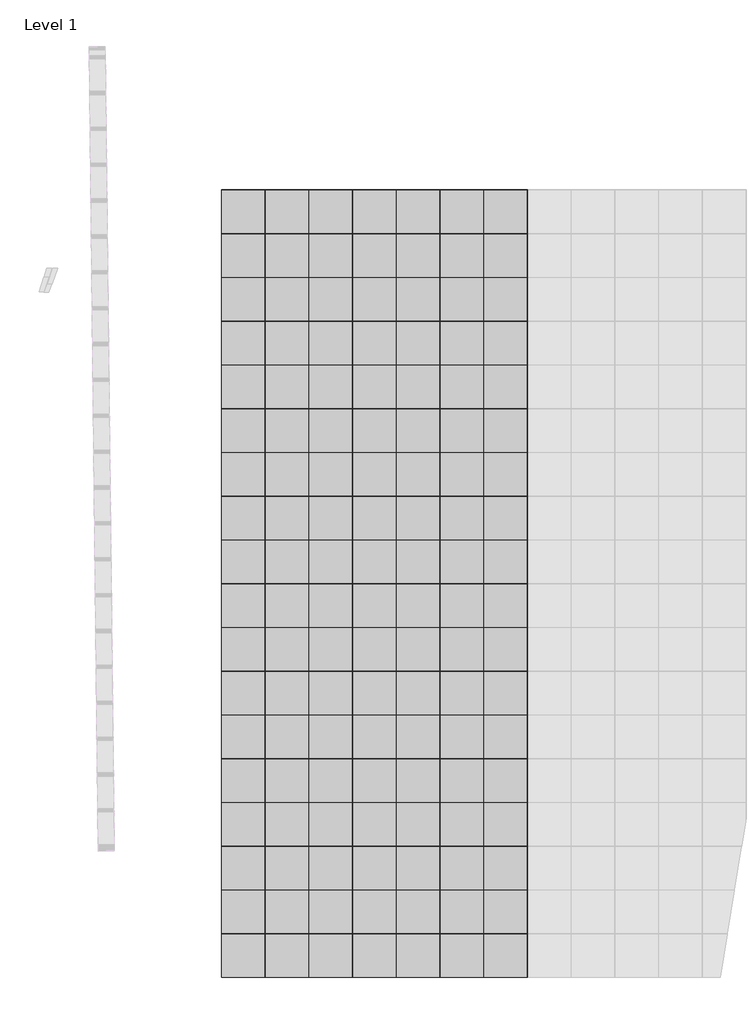
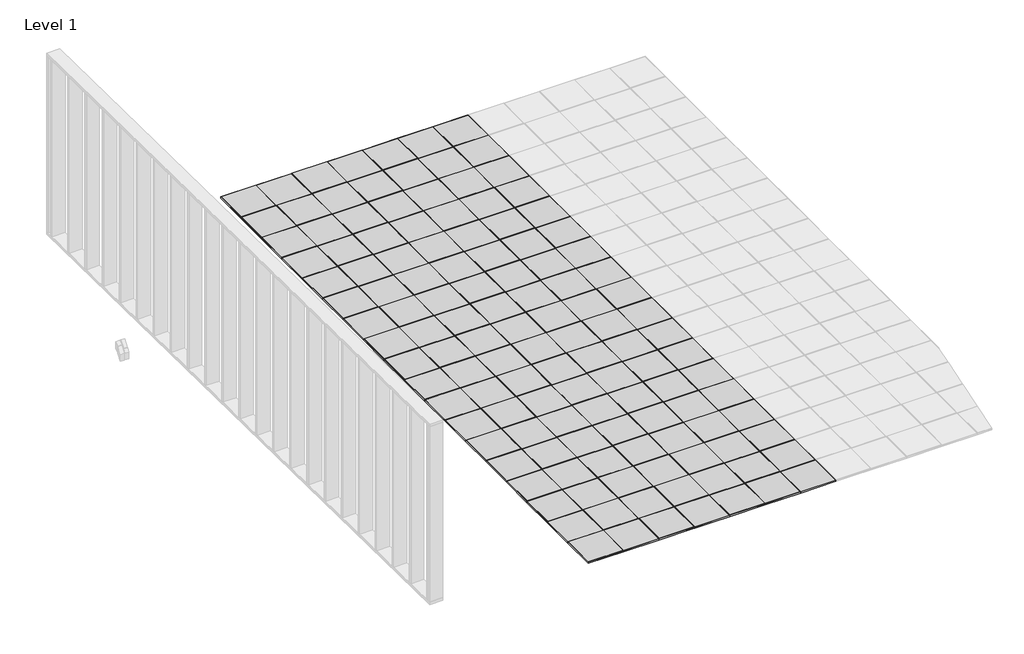
# One storey, part 1 of 18: 126 plates.
"""IFC4 building model written with IfcOpenShell, lengths in millimetres."""

import ifcopenshell
import ifcopenshell.guid

model = None  # the IFC model being written
_history = None  # IfcOwnerHistory: only IFC2X3 demands one
_inside = {}  # id of a spatial element -> (the spatial element, [elements in it])
_under = {}  # id of a project, library or spatial element -> (it, [spatial elements below it])
_declared = {}  # id of a project -> (the project, [libraries it declares])
_typed = {}  # id of a type object -> (the type object, [elements of that type])
_made_of = {}  # id of a material, layer set ... -> (it, [elements and type objects made of it])


def new_model(schema):
    """Start an empty IFC model of exactly this schema.

    Asked for "IFC4X3", IfcOpenShell would pick the latest addendum, in which some entities
    have other attributes; the version numbers below select the first issue.
    IFC2X3 requires an IfcOwnerHistory on every rooted entity: one is made here for all.
    """
    global model, _history
    if schema == "IFC4X3":
        model = ifcopenshell.file(schema_version=(4, 3, 0, 0))
    else:
        model = ifcopenshell.file(schema=schema)
    _inside.clear()
    _under.clear()
    _declared.clear()
    _typed.clear()
    _made_of.clear()
    _history = None
    if model.schema == "IFC2X3":
        org = make("IfcOrganization", Name="unknown")
        user = make(
            "IfcPersonAndOrganization",
            ThePerson=make("IfcPerson", FamilyName="unknown"),
            TheOrganization=org,
        )
        app = make(
            "IfcApplication",
            ApplicationDeveloper=org,
            Version="unknown",
            ApplicationFullName="unknown",
            ApplicationIdentifier="unknown",
        )
        _history = make(
            "IfcOwnerHistory",
            OwningUser=user,
            OwningApplication=app,
            ChangeAction="ADDED",
            CreationDate=0,
        )
    return model


def make(cls, **values):
    """One entity of the class cls with the attributes given. An attribute that is None is left unset."""
    return model.create_entity(
        cls, **{name: value for name, value in values.items() if value is not None}
    )


def rooted(cls, **values):
    """An entity with a GlobalId (a new one), such as an element, a storey or a relation."""
    return make(cls, GlobalId=ifcopenshell.guid.new(), OwnerHistory=_history, **values)


def si_unit(unit_type, name, prefix=None):
    """IfcSIUnit, for example si_unit("LENGTHUNIT", "METRE", prefix="MILLI")."""
    return make("IfcSIUnit", UnitType=unit_type, Prefix=prefix, Name=name)


def assignment(units):
    """IfcUnitAssignment: the units of a project."""
    return None if units is None else make("IfcUnitAssignment", Units=units)


def point(xyz):
    """IfcCartesianPoint."""
    return None if xyz is None else make("IfcCartesianPoint", Coordinates=xyz)


def direction(xyz):
    """IfcDirection."""
    return None if xyz is None else make("IfcDirection", DirectionRatios=xyz)


def frame(location, z_axis=None, x_axis=None):
    """IfcAxis2Placement3D, a coordinate frame: its origin and axes. An axis left out is left unset."""
    return make(
        "IfcAxis2Placement3D",
        Location=point(location),
        Axis=direction(z_axis),
        RefDirection=direction(x_axis),
    )


def origin():
    """The frame at (0, 0, 0) with its axes left unset."""
    return frame((0.0, 0.0, 0.0))


def origin_with_axes():
    """The frame at (0, 0, 0) with the z axis (0, 0, 1) and the x axis (1, 0, 0) written out."""
    return frame((0.0, 0.0, 0.0), z_axis=(0.0, 0.0, 1.0), x_axis=(1.0, 0.0, 0.0))


def place(relative_to, where):
    """IfcLocalPlacement: puts the frame where relative to a parent placement (None: the world)."""
    return make(
        "IfcLocalPlacement", PlacementRelTo=relative_to, RelativePlacement=where
    )


def context(
    kind, dimensions, precision=None, world=None, true_north=None, identifier=None
):
    """IfcGeometricRepresentationContext, for example the 3D "Model" context."""
    return make(
        "IfcGeometricRepresentationContext",
        ContextIdentifier=identifier,
        ContextType=kind,
        CoordinateSpaceDimension=dimensions,
        Precision=precision,
        WorldCoordinateSystem=world,
        TrueNorth=true_north,
    )


def project(units=None, contexts=None):
    """IfcProject with its units and contexts."""
    return rooted(
        "IfcProject",
        Name="project",
        RepresentationContexts=contexts,
        UnitsInContext=assignment(units),
    )


def spatial(cls, under=None, at=None, **own):
    """A site, building, storey or space (cls), placed at a placement, below another one or the project."""
    s = rooted(cls, ObjectPlacement=at, **own)
    if under is not None:
        _under.setdefault(under.id(), (under, []))[1].append(s)
    return s


def polyline(points):
    """IfcPolyline through the points."""
    return make("IfcPolyline", Points=[point(p) for p in points])


def outline(outer, holes=None, kind="AREA"):
    """IfcArbitraryClosedProfileDef: a profile drawn as a closed curve; with holes, ...WithVoids."""
    if holes is None:
        return make("IfcArbitraryClosedProfileDef", ProfileType=kind, OuterCurve=outer)
    return make(
        "IfcArbitraryProfileDefWithVoids",
        ProfileType=kind,
        OuterCurve=outer,
        InnerCurves=holes,
    )


def extrude(swept, where, along, depth):
    """IfcExtrudedAreaSolid: the profile swept, set in the frame where, extruded along a direction by depth."""
    return make(
        "IfcExtrudedAreaSolid",
        SweptArea=swept,
        Position=where,
        ExtrudedDirection=direction(along),
        Depth=depth,
    )


def shape(context_of_items, identifier, shape_type, items):
    """IfcShapeRepresentation: the items that make up one representation, for example the "Body"."""
    return make(
        "IfcShapeRepresentation",
        ContextOfItems=context_of_items,
        RepresentationIdentifier=identifier,
        RepresentationType=shape_type,
        Items=items,
    )


def source(mapping_origin, context_of_items, identifier, shape_type, items):
    """IfcRepresentationMap: a shape defined once, which mapped items show again and again."""
    return make(
        "IfcRepresentationMap",
        MappingOrigin=mapping_origin,
        MappedRepresentation=shape(context_of_items, identifier, shape_type, items),
    )


def transform(
    local_origin,
    x_axis=None,
    y_axis=None,
    z_axis=None,
    scale=None,
    scale2=None,
    scale3=None,
    uniform=True,
):
    """IfcCartesianTransformationOperator3D, or its non-uniform kind. x_axis, y_axis, z_axis: its Axis1, 2, 3."""
    if uniform:
        return make(
            "IfcCartesianTransformationOperator3D",
            Axis1=direction(x_axis),
            Axis2=direction(y_axis),
            LocalOrigin=point(local_origin),
            Scale=scale,
            Axis3=direction(z_axis),
        )
    return make(
        "IfcCartesianTransformationOperator3DnonUniform",
        Axis1=direction(x_axis),
        Axis2=direction(y_axis),
        LocalOrigin=point(local_origin),
        Scale=scale,
        Axis3=direction(z_axis),
        Scale2=scale2,
        Scale3=scale3,
    )


def mapped(mapping_source, mapping_target):
    """IfcMappedItem: shows the shape of a source again, moved by a transform."""
    return make(
        "IfcMappedItem", MappingSource=mapping_source, MappingTarget=mapping_target
    )


def made_of(thing, what):
    """Note that an element or type object is made of a material, layer set ...; save() writes the relation."""
    if what is not None:
        _made_of.setdefault(what.id(), (what, []))[1].append(thing)
    return thing


def element(
    cls,
    number,
    at=None,
    inside=None,
    cuts=None,
    type_object=None,
    material=None,
    context=None,
    identifier="Body",
    shape_type=None,
    held_by="IfcProductDefinitionShape",
    body=None,
    shapes=None,
    **own,
):
    """One element of the class cls, such as IfcWall. Its Tag is "e" and its number.

    at: its placement. inside: the storey or other place that contains it. cuts: it is an
    opening in that element (IfcRelVoidsElement). A single representation is given by context,
    identifier, shape_type and body (its items); several are given by shapes. held_by: the class
    of the entity that holds the representations. save() writes the other relations.
    """
    e = rooted(cls, Tag="e%d" % number, ObjectPlacement=at, **own)
    if body is not None:
        shapes = [shape(context, identifier, shape_type, body)]
    if shapes is not None:
        e.Representation = make(held_by, Representations=shapes)
    if inside is not None:
        _inside.setdefault(inside.id(), (inside, []))[1].append(e)
    if cuts is not None:
        rooted(
            "IfcRelVoidsElement", RelatingBuildingElement=cuts, RelatedOpeningElement=e
        )
    if type_object is not None:
        _typed.setdefault(type_object.id(), (type_object, []))[1].append(e)
    return made_of(e, material)


def aggregate(whole, parts):
    """IfcRelAggregates: a whole, such as a stair, and the parts it consists of."""
    return rooted("IfcRelAggregates", RelatingObject=whole, RelatedObjects=parts)


def save(model, path):
    """Write the relations noted so far, then the file.

    IfcRelAggregates (storeys below a building ...), IfcRelContainedInSpatialStructure (elements
    in a storey), IfcRelDefinesByType, IfcRelAssociatesMaterial and IfcRelDeclares: one each for
    every whole, place, type object, material and project.
    """
    for whole, parts in _under.values():
        aggregate(whole, parts)
    for where, things in _inside.values():
        rooted(
            "IfcRelContainedInSpatialStructure",
            RelatedElements=things,
            RelatingStructure=where,
        )
    for kind, things in _typed.values():
        rooted("IfcRelDefinesByType", RelatedObjects=things, RelatingType=kind)
    for what, things in _made_of.values():
        rooted("IfcRelAssociatesMaterial", RelatedObjects=things, RelatingMaterial=what)
    for by, libraries in _declared.values():
        rooted("IfcRelDeclares", RelatingContext=by, RelatedDefinitions=libraries)
    model.write(path)


def type_1_8eb2385c(model_context):
    return source(origin(), model_context, "Body", "SweptSolid", [
        extrude(outline(polyline([(1000.0, 500.0), (500.0, 500.0), (500.0, 1000.0), (1000.0, 1000.0), (1000.0, 500.0)]), holes=[polyline([(995.0, 995.0), (505.0, 995.0), (505.0, 505.0), (995.0, 505.0), (995.0, 995.0)])]), origin_with_axes(), (0.0, 0.0, 1.0), 18.0),
        extrude(outline(polyline([(505.0, 995.0), (995.0, 995.0), (995.0, 505.0), (505.0, 505.0), (505.0, 995.0)])), origin_with_axes(), (0.0, 0.0, 1.0), 20.0),
    ])


model = new_model("IFC4")

# Units and contexts
model_context = context("Model", 3, world=origin())
ifc_project = project(units=[si_unit("LENGTHUNIT", "METRE", prefix="MILLI")], contexts=[model_context])

# Site, building, storey
site = spatial("IfcSite", under=ifc_project)
building = spatial("IfcBuilding", under=site)
storey = spatial("IfcBuildingStorey", under=building, Name="Level 1", Elevation=0.0)

# Plates
placement = place(None, origin())
element("IfcPlate", 1, ObjectType="00_CPA_tegel : Type 1", at=placement, inside=storey, context=model_context, shape_type="SweptSolid", body=[
    extrude(outline(polyline([(-1945.6207016, -8414.3640992), (-1455.6207017, -8414.373882), (-1455.6304844, -8904.3738819), (-1945.6304843, -8904.3640991), (-1945.6207016, -8414.3640992)])), frame((0.0, 0.0, 1000.0), z_axis=(0.0, 0.0, 1.0), x_axis=(1.0, 0.0, 0.0)), (0.0, 0.0, 1.0), 20.0),
    extrude(outline(polyline([(-1450.6305843, -8909.3739817), (-1950.6305842, -8909.3639993), (-1950.6206017, -8409.3639994), (-1450.6206018, -8409.3739818), (-1450.6305843, -8909.3739817)]), holes=[polyline([(-1455.6207017, -8414.373882), (-1945.6207016, -8414.3640992), (-1945.6304843, -8904.3640991), (-1455.6304844, -8904.3738819), (-1455.6207017, -8414.373882)])]), frame((0.0, 0.0, 1000.0), z_axis=(0.0, 0.0, 1.0), x_axis=(1.0, 0.0, 0.0)), (0.0, 0.0, 1.0), 18.0),
])
type_1_shape = type_1_8eb2385c(model_context)
element("IfcPlate", 2, ObjectType="00_CPA_tegel : Type 1", at=placement, inside=storey, context=model_context, shape_type="MappedRepresentation", body=[
    mapped(type_1_shape, transform((-2950.8002853, -17409.3440327, 1000.0), x_axis=(0.9999999998007024, -1.9964866676325244e-05, 0.0), y_axis=(1.9964866676325244e-05, 0.9999999998007024, 0.0), z_axis=(0.0, 0.0, 1.0))),
])
element("IfcPlate", 3, ObjectType="00_CPA_tegel : Type 1", at=placement, inside=storey, context=model_context, shape_type="MappedRepresentation", body=[
    mapped(type_1_shape, transform((-2450.8002854, -17409.3540152, 1000.0), x_axis=(0.9999999998007023, -1.9964866675492576e-05, 0.0), y_axis=(1.9964866675492576e-05, 0.9999999998007023, 0.0), z_axis=(0.0, 0.0, 1.0))),
])
element("IfcPlate", 4, ObjectType="00_CPA_tegel : Type 1", at=placement, inside=storey, context=model_context, shape_type="MappedRepresentation", body=[
    mapped(type_1_shape, transform((-1950.8002855, -17409.3639976, 1000.0), x_axis=(0.9999999998007023, -1.9964866675492576e-05, 0.0), y_axis=(1.9964866675492576e-05, 0.9999999998007023, 0.0), z_axis=(0.0, 0.0, 1.0))),
])
element("IfcPlate", 5, ObjectType="00_CPA_tegel : Type 1", at=placement, inside=storey, context=model_context, shape_type="MappedRepresentation", body=[
    mapped(type_1_shape, transform((-1450.8002856, -17409.37398, 1000.0), x_axis=(0.9999999998007022, -1.9964866674881954e-05, 0.0), y_axis=(1.9964866674881954e-05, 0.9999999998007022, 0.0), z_axis=(0.0, 0.0, 1.0))),
])
element("IfcPlate", 6, ObjectType="00_CPA_tegel : Type 1", at=placement, inside=storey, context=model_context, shape_type="MappedRepresentation", body=[
    mapped(type_1_shape, transform((-950.8002857, -17409.3839625, 1000.0), x_axis=(0.9999999998007023, -1.9964866675492576e-05, 0.0), y_axis=(1.9964866675492576e-05, 0.9999999998007023, 0.0), z_axis=(0.0, 0.0, 1.0))),
])
element("IfcPlate", 7, ObjectType="00_CPA_tegel : Type 1", at=placement, inside=storey, context=model_context, shape_type="MappedRepresentation", body=[
    mapped(type_1_shape, transform((-2950.7903029, -16909.3440328, 1000.0), x_axis=(0.9999999998007023, -1.9964866675492576e-05, 0.0), y_axis=(1.9964866675492576e-05, 0.9999999998007023, 0.0), z_axis=(0.0, 0.0, 1.0))),
])
element("IfcPlate", 8, ObjectType="00_CPA_tegel : Type 1", at=placement, inside=storey, context=model_context, shape_type="MappedRepresentation", body=[
    mapped(type_1_shape, transform((-2450.790303, -16909.3540152, 1000.0), x_axis=(0.9999999998007022, -1.9964866674881954e-05, 0.0), y_axis=(1.9964866674881954e-05, 0.9999999998007022, 0.0), z_axis=(0.0, 0.0, 1.0))),
])
element("IfcPlate", 9, ObjectType="00_CPA_tegel : Type 1", at=placement, inside=storey, context=model_context, shape_type="MappedRepresentation", body=[
    mapped(type_1_shape, transform((-1950.7903031, -16909.3639977, 1000.0), x_axis=(0.9999999998007022, -1.9964866674881954e-05, 0.0), y_axis=(1.9964866674881954e-05, 0.9999999998007022, 0.0), z_axis=(0.0, 0.0, 1.0))),
])
element("IfcPlate", 10, ObjectType="00_CPA_tegel : Type 1", at=placement, inside=storey, context=model_context, shape_type="MappedRepresentation", body=[
    mapped(type_1_shape, transform((-1450.7903032, -16909.3739801, 1000.0), x_axis=(0.9999999998007022, -1.9964866674881954e-05, 0.0), y_axis=(1.9964866674881954e-05, 0.9999999998007022, 0.0), z_axis=(0.0, 0.0, 1.0))),
])
element("IfcPlate", 11, ObjectType="00_CPA_tegel : Type 1", at=placement, inside=storey, context=model_context, shape_type="MappedRepresentation", body=[
    mapped(type_1_shape, transform((-950.7903033, -16909.3839625, 1000.0), x_axis=(0.9999999998007022, -1.9964866674881954e-05, 0.0), y_axis=(1.9964866674881954e-05, 0.9999999998007022, 0.0), z_axis=(0.0, 0.0, 1.0))),
])
element("IfcPlate", 12, ObjectType="00_CPA_tegel : Type 1", at=placement, inside=storey, context=model_context, shape_type="MappedRepresentation", body=[
    mapped(type_1_shape, transform((-2950.7803205, -16409.3440329, 1000.0), x_axis=(0.9999999998007022, -1.9964866674881954e-05, 0.0), y_axis=(1.9964866674881954e-05, 0.9999999998007022, 0.0), z_axis=(0.0, 0.0, 1.0))),
])
element("IfcPlate", 13, ObjectType="00_CPA_tegel : Type 1", at=placement, inside=storey, context=model_context, shape_type="MappedRepresentation", body=[
    mapped(type_1_shape, transform((-2450.7803206, -16409.3540153, 1000.0), x_axis=(0.9999999998007022, -1.9964866674881954e-05, 0.0), y_axis=(1.9964866674881954e-05, 0.9999999998007022, 0.0), z_axis=(0.0, 0.0, 1.0))),
])
element("IfcPlate", 14, ObjectType="00_CPA_tegel : Type 1", at=placement, inside=storey, context=model_context, shape_type="MappedRepresentation", body=[
    mapped(type_1_shape, transform((-1950.7803207, -16409.3639978, 1000.0), x_axis=(0.9999999998007022, -1.9964866674881954e-05, 0.0), y_axis=(1.9964866674881954e-05, 0.9999999998007022, 0.0), z_axis=(0.0, 0.0, 1.0))),
])
element("IfcPlate", 15, ObjectType="00_CPA_tegel : Type 1", at=placement, inside=storey, context=model_context, shape_type="MappedRepresentation", body=[
    mapped(type_1_shape, transform((-1450.7803208, -16409.3739802, 1000.0), x_axis=(0.9999999998007021, -1.996486667421582e-05, 0.0), y_axis=(1.996486667421582e-05, 0.9999999998007021, 0.0), z_axis=(0.0, 0.0, 1.0))),
])
element("IfcPlate", 16, ObjectType="00_CPA_tegel : Type 1", at=placement, inside=storey, context=model_context, shape_type="MappedRepresentation", body=[
    mapped(type_1_shape, transform((-950.7803209, -16409.3839626, 1000.0), x_axis=(0.9999999998007022, -1.9964866674881954e-05, 0.0), y_axis=(1.9964866674881954e-05, 0.9999999998007022, 0.0), z_axis=(0.0, 0.0, 1.0))),
])
element("IfcPlate", 17, ObjectType="00_CPA_tegel : Type 1", at=placement, inside=storey, context=model_context, shape_type="MappedRepresentation", body=[
    mapped(type_1_shape, transform((-2950.770338, -15909.344033, 1000.0), x_axis=(0.9999999998007024, -1.9964866676325244e-05, 0.0), y_axis=(1.9964866676325244e-05, 0.9999999998007024, 0.0), z_axis=(0.0, 0.0, 1.0))),
])
element("IfcPlate", 18, ObjectType="00_CPA_tegel : Type 1", at=placement, inside=storey, context=model_context, shape_type="MappedRepresentation", body=[
    mapped(type_1_shape, transform((-2450.7703381, -15909.3540154, 1000.0), x_axis=(0.9999999998007024, -1.9964866676325244e-05, 0.0), y_axis=(1.9964866676325244e-05, 0.9999999998007024, 0.0), z_axis=(0.0, 0.0, 1.0))),
])
element("IfcPlate", 19, ObjectType="00_CPA_tegel : Type 1", at=placement, inside=storey, context=model_context, shape_type="MappedRepresentation", body=[
    mapped(type_1_shape, transform((-1950.7703382, -15909.3639979, 1000.0), x_axis=(0.9999999998007024, -1.9964866676325244e-05, 0.0), y_axis=(1.9964866676325244e-05, 0.9999999998007024, 0.0), z_axis=(0.0, 0.0, 1.0))),
])
element("IfcPlate", 20, ObjectType="00_CPA_tegel : Type 1", at=placement, inside=storey, context=model_context, shape_type="MappedRepresentation", body=[
    mapped(type_1_shape, transform((-1450.7703383, -15909.3739803, 1000.0), x_axis=(0.9999999998007023, -1.9964866675492576e-05, 0.0), y_axis=(1.9964866675492576e-05, 0.9999999998007023, 0.0), z_axis=(0.0, 0.0, 1.0))),
])
element("IfcPlate", 21, ObjectType="00_CPA_tegel : Type 1", at=placement, inside=storey, context=model_context, shape_type="MappedRepresentation", body=[
    mapped(type_1_shape, transform((-950.7703384, -15909.3839627, 1000.0), x_axis=(0.9999999998007024, -1.9964866676325244e-05, 0.0), y_axis=(1.9964866676325244e-05, 0.9999999998007024, 0.0), z_axis=(0.0, 0.0, 1.0))),
])
element("IfcPlate", 22, ObjectType="00_CPA_tegel : Type 1", at=placement, inside=storey, context=model_context, shape_type="MappedRepresentation", body=[
    mapped(type_1_shape, transform((-2950.7603556, -15409.3440331, 1000.0), x_axis=(0.9999999998007023, -1.9964866675492576e-05, 0.0), y_axis=(1.9964866675492576e-05, 0.9999999998007023, 0.0), z_axis=(0.0, 0.0, 1.0))),
])
element("IfcPlate", 23, ObjectType="00_CPA_tegel : Type 1", at=placement, inside=storey, context=model_context, shape_type="MappedRepresentation", body=[
    mapped(type_1_shape, transform((-2450.7603557, -15409.3540155, 1000.0), x_axis=(0.9999999998007023, -1.9964866675492576e-05, 0.0), y_axis=(1.9964866675492576e-05, 0.9999999998007023, 0.0), z_axis=(0.0, 0.0, 1.0))),
])
element("IfcPlate", 24, ObjectType="00_CPA_tegel : Type 1", at=placement, inside=storey, context=model_context, shape_type="MappedRepresentation", body=[
    mapped(type_1_shape, transform((-1950.7603558, -15409.363998, 1000.0), x_axis=(0.9999999998007023, -1.9964866675492576e-05, 0.0), y_axis=(1.9964866675492576e-05, 0.9999999998007023, 0.0), z_axis=(0.0, 0.0, 1.0))),
])
element("IfcPlate", 25, ObjectType="00_CPA_tegel : Type 1", at=placement, inside=storey, context=model_context, shape_type="MappedRepresentation", body=[
    mapped(type_1_shape, transform((-1450.7603559, -15409.3739804, 1000.0), x_axis=(0.9999999998007022, -1.9964866674881954e-05, 0.0), y_axis=(1.9964866674881954e-05, 0.9999999998007022, 0.0), z_axis=(0.0, 0.0, 1.0))),
])
element("IfcPlate", 26, ObjectType="00_CPA_tegel : Type 1", at=placement, inside=storey, context=model_context, shape_type="MappedRepresentation", body=[
    mapped(type_1_shape, transform((-950.760356, -15409.3839628, 1000.0), x_axis=(0.9999999998007023, -1.9964866675492576e-05, 0.0), y_axis=(1.9964866675492576e-05, 0.9999999998007023, 0.0), z_axis=(0.0, 0.0, 1.0))),
])
element("IfcPlate", 27, ObjectType="00_CPA_tegel : Type 1", at=placement, inside=storey, context=model_context, shape_type="MappedRepresentation", body=[
    mapped(type_1_shape, transform((-2950.7503732, -14909.3440332, 1000.0), x_axis=(0.9999999998007023, -1.9964866675492576e-05, 0.0), y_axis=(1.9964866675492576e-05, 0.9999999998007023, 0.0), z_axis=(0.0, 0.0, 1.0))),
])
element("IfcPlate", 28, ObjectType="00_CPA_tegel : Type 1", at=placement, inside=storey, context=model_context, shape_type="MappedRepresentation", body=[
    mapped(type_1_shape, transform((-2450.7503733, -14909.3540156, 1000.0), x_axis=(0.9999999998007024, -1.9964866676991377e-05, 0.0), y_axis=(1.9964866676991377e-05, 0.9999999998007024, 0.0), z_axis=(0.0, 0.0, 1.0))),
])
element("IfcPlate", 29, ObjectType="00_CPA_tegel : Type 1", at=placement, inside=storey, context=model_context, shape_type="MappedRepresentation", body=[
    mapped(type_1_shape, transform((-1950.7503734, -14909.3639981, 1000.0), x_axis=(0.9999999998007023, -1.9964866675492576e-05, 0.0), y_axis=(1.9964866675492576e-05, 0.9999999998007023, 0.0), z_axis=(0.0, 0.0, 1.0))),
])
element("IfcPlate", 30, ObjectType="00_CPA_tegel : Type 1", at=placement, inside=storey, context=model_context, shape_type="MappedRepresentation", body=[
    mapped(type_1_shape, transform((-1450.7503735, -14909.3739805, 1000.0), x_axis=(0.9999999998007024, -1.9964866676991377e-05, 0.0), y_axis=(1.9964866676991377e-05, 0.9999999998007024, 0.0), z_axis=(0.0, 0.0, 1.0))),
])
element("IfcPlate", 31, ObjectType="00_CPA_tegel : Type 1", at=placement, inside=storey, context=model_context, shape_type="MappedRepresentation", body=[
    mapped(type_1_shape, transform((-950.7503736, -14909.3839629, 1000.0), x_axis=(0.9999999998007024, -1.9964866676991377e-05, 0.0), y_axis=(1.9964866676991377e-05, 0.9999999998007024, 0.0), z_axis=(0.0, 0.0, 1.0))),
])
element("IfcPlate", 32, ObjectType="00_CPA_tegel : Type 1", at=placement, inside=storey, context=model_context, shape_type="MappedRepresentation", body=[
    mapped(type_1_shape, transform((-2950.7403907, -14409.3440333, 1000.0), x_axis=(0.9999999998007023, -1.9964866675492576e-05, 0.0), y_axis=(1.9964866675492576e-05, 0.9999999998007023, 0.0), z_axis=(0.0, 0.0, 1.0))),
])
element("IfcPlate", 33, ObjectType="00_CPA_tegel : Type 1", at=placement, inside=storey, context=model_context, shape_type="MappedRepresentation", body=[
    mapped(type_1_shape, transform((-2450.7403908, -14409.3540157, 1000.0), x_axis=(0.9999999998007024, -1.9964866676325244e-05, 0.0), y_axis=(1.9964866676325244e-05, 0.9999999998007024, 0.0), z_axis=(0.0, 0.0, 1.0))),
])
element("IfcPlate", 34, ObjectType="00_CPA_tegel : Type 1", at=placement, inside=storey, context=model_context, shape_type="MappedRepresentation", body=[
    mapped(type_1_shape, transform((-1950.7403909, -14409.3639982, 1000.0), x_axis=(0.9999999998007022, -1.9964866674881954e-05, 0.0), y_axis=(1.9964866674881954e-05, 0.9999999998007022, 0.0), z_axis=(0.0, 0.0, 1.0))),
])
element("IfcPlate", 35, ObjectType="00_CPA_tegel : Type 1", at=placement, inside=storey, context=model_context, shape_type="MappedRepresentation", body=[
    mapped(type_1_shape, transform((-1450.740391, -14409.3739806, 1000.0), x_axis=(0.9999999998007023, -1.9964866675492576e-05, 0.0), y_axis=(1.9964866675492576e-05, 0.9999999998007023, 0.0), z_axis=(0.0, 0.0, 1.0))),
])
element("IfcPlate", 36, ObjectType="00_CPA_tegel : Type 1", at=placement, inside=storey, context=model_context, shape_type="MappedRepresentation", body=[
    mapped(type_1_shape, transform((-950.7403911, -14409.383963, 1000.0), x_axis=(0.9999999998007023, -1.9964866675492576e-05, 0.0), y_axis=(1.9964866675492576e-05, 0.9999999998007023, 0.0), z_axis=(0.0, 0.0, 1.0))),
])
element("IfcPlate", 37, ObjectType="00_CPA_tegel : Type 1", at=placement, inside=storey, context=model_context, shape_type="MappedRepresentation", body=[
    mapped(type_1_shape, transform((-2950.7304083, -13909.3440334, 1000.0), x_axis=(0.9999999998007024, -1.9964866676325244e-05, 0.0), y_axis=(1.9964866676325244e-05, 0.9999999998007024, 0.0), z_axis=(0.0, 0.0, 1.0))),
])
element("IfcPlate", 38, ObjectType="00_CPA_tegel : Type 1", at=placement, inside=storey, context=model_context, shape_type="MappedRepresentation", body=[
    mapped(type_1_shape, transform((-2450.7304084, -13909.3540158, 1000.0), x_axis=(0.9999999998007022, -1.9964866676935866e-05, 0.0), y_axis=(1.9964866676935866e-05, 0.9999999998007022, 0.0), z_axis=(0.0, 0.0, 1.0))),
])
element("IfcPlate", 39, ObjectType="00_CPA_tegel : Type 1", at=placement, inside=storey, context=model_context, shape_type="MappedRepresentation", body=[
    mapped(type_1_shape, transform((-1950.7304085, -13909.3639983, 1000.0), x_axis=(0.9999999998007024, -1.9964866676991377e-05, 0.0), y_axis=(1.9964866676991377e-05, 0.9999999998007024, 0.0), z_axis=(0.0, 0.0, 1.0))),
])
element("IfcPlate", 40, ObjectType="00_CPA_tegel : Type 1", at=placement, inside=storey, context=model_context, shape_type="MappedRepresentation", body=[
    mapped(type_1_shape, transform((-1450.7304086, -13909.3739807, 1000.0), x_axis=(0.9999999998007023, -1.9964866675492576e-05, 0.0), y_axis=(1.9964866675492576e-05, 0.9999999998007023, 0.0), z_axis=(0.0, 0.0, 1.0))),
])
element("IfcPlate", 41, ObjectType="00_CPA_tegel : Type 1", at=placement, inside=storey, context=model_context, shape_type="MappedRepresentation", body=[
    mapped(type_1_shape, transform((-950.7304087, -13909.3839631, 1000.0), x_axis=(0.9999999998007023, -1.9964866675492576e-05, 0.0), y_axis=(1.9964866675492576e-05, 0.9999999998007023, 0.0), z_axis=(0.0, 0.0, 1.0))),
])
element("IfcPlate", 42, ObjectType="00_CPA_tegel : Type 1", at=placement, inside=storey, context=model_context, shape_type="MappedRepresentation", body=[
    mapped(type_1_shape, transform((-2950.7204259, -13409.3440335, 1000.0), x_axis=(0.9999999998007023, -1.9964866675492576e-05, 0.0), y_axis=(1.9964866675492576e-05, 0.9999999998007023, 0.0), z_axis=(0.0, 0.0, 1.0))),
])
element("IfcPlate", 43, ObjectType="00_CPA_tegel : Type 1", at=placement, inside=storey, context=model_context, shape_type="MappedRepresentation", body=[
    mapped(type_1_shape, transform((-2450.720426, -13409.3540159, 1000.0), x_axis=(0.9999999998007022, -1.9964866677602e-05, 0.0), y_axis=(1.9964866677602e-05, 0.9999999998007022, 0.0), z_axis=(0.0, 0.0, 1.0))),
])
element("IfcPlate", 44, ObjectType="00_CPA_tegel : Type 1", at=placement, inside=storey, context=model_context, shape_type="MappedRepresentation", body=[
    mapped(type_1_shape, transform((-1950.7204261, -13409.3639984, 1000.0), x_axis=(0.9999999998007024, -1.9964866676991377e-05, 0.0), y_axis=(1.9964866676991377e-05, 0.9999999998007024, 0.0), z_axis=(0.0, 0.0, 1.0))),
])
element("IfcPlate", 45, ObjectType="00_CPA_tegel : Type 1", at=placement, inside=storey, context=model_context, shape_type="MappedRepresentation", body=[
    mapped(type_1_shape, transform((-1450.7204262, -13409.3739808, 1000.0), x_axis=(0.9999999998007022, -1.996486667416031e-05, 0.0), y_axis=(1.996486667416031e-05, 0.9999999998007022, 0.0), z_axis=(0.0, 0.0, 1.0))),
])
element("IfcPlate", 46, ObjectType="00_CPA_tegel : Type 1", at=placement, inside=storey, context=model_context, shape_type="MappedRepresentation", body=[
    mapped(type_1_shape, transform((-950.7204263, -13409.3839632, 1000.0), x_axis=(0.9999999998007024, -1.9964866676991377e-05, 0.0), y_axis=(1.9964866676991377e-05, 0.9999999998007024, 0.0), z_axis=(0.0, 0.0, 1.0))),
])
element("IfcPlate", 47, ObjectType="00_CPA_tegel : Type 1", at=placement, inside=storey, context=model_context, shape_type="MappedRepresentation", body=[
    mapped(type_1_shape, transform((-950.7104438, -12909.3839633, 1000.0), x_axis=(0.9999999998007023, -1.9964866675492576e-05, 0.0), y_axis=(1.9964866675492576e-05, 0.9999999998007023, 0.0), z_axis=(0.0, 0.0, 1.0))),
])
element("IfcPlate", 48, ObjectType="00_CPA_tegel : Type 1", at=placement, inside=storey, context=model_context, shape_type="MappedRepresentation", body=[
    mapped(type_1_shape, transform((-1450.7104437, -12909.3739809, 1000.0), x_axis=(0.9999999998007022, -1.996486667416031e-05, 0.0), y_axis=(1.996486667416031e-05, 0.9999999998007022, 0.0), z_axis=(0.0, 0.0, 1.0))),
])
element("IfcPlate", 49, ObjectType="00_CPA_tegel : Type 1", at=placement, inside=storey, context=model_context, shape_type="MappedRepresentation", body=[
    mapped(type_1_shape, transform((-2950.7104434, -12909.3440336, 1000.0), x_axis=(0.9999999998007024, -1.9964866676325244e-05, 0.0), y_axis=(1.9964866676325244e-05, 0.9999999998007024, 0.0), z_axis=(0.0, 0.0, 1.0))),
])
element("IfcPlate", 50, ObjectType="00_CPA_tegel : Type 1", at=placement, inside=storey, context=model_context, shape_type="MappedRepresentation", body=[
    mapped(type_1_shape, transform((-2450.7104435, -12909.354016, 1000.0), x_axis=(0.9999999998007022, -1.9964866674881954e-05, 0.0), y_axis=(1.9964866674881954e-05, 0.9999999998007022, 0.0), z_axis=(0.0, 0.0, 1.0))),
])
element("IfcPlate", 51, ObjectType="00_CPA_tegel : Type 1", at=placement, inside=storey, context=model_context, shape_type="MappedRepresentation", body=[
    mapped(type_1_shape, transform((-1950.7104436, -12909.3639985, 1000.0), x_axis=(0.9999999998007022, -1.9964866678934268e-05, 0.0), y_axis=(1.9964866678934268e-05, 0.9999999998007022, 0.0), z_axis=(0.0, 0.0, 1.0))),
])
element("IfcPlate", 52, ObjectType="00_CPA_tegel : Type 1", at=placement, inside=storey, context=model_context, shape_type="MappedRepresentation", body=[
    mapped(type_1_shape, transform((-950.7004614, -12409.3839634, 1000.0), x_axis=(0.9999999998007022, -1.996486667416031e-05, 0.0), y_axis=(1.996486667416031e-05, 0.9999999998007022, 0.0), z_axis=(0.0, 0.0, 1.0))),
])
element("IfcPlate", 53, ObjectType="00_CPA_tegel : Type 1", at=placement, inside=storey, context=model_context, shape_type="MappedRepresentation", body=[
    mapped(type_1_shape, transform((-450.8002858, -17409.3939449, 1000.0), x_axis=(0.9999999998007022, -1.9964866674881954e-05, 0.0), y_axis=(1.9964866674881954e-05, 0.9999999998007022, 0.0), z_axis=(0.0, 0.0, 1.0))),
])
element("IfcPlate", 54, ObjectType="00_CPA_tegel : Type 1", at=placement, inside=storey, context=model_context, shape_type="MappedRepresentation", body=[
    mapped(type_1_shape, transform((-450.7903034, -16909.393945, 1000.0), x_axis=(0.9999999998007023, -1.9964866675492576e-05, 0.0), y_axis=(1.9964866675492576e-05, 0.9999999998007023, 0.0), z_axis=(0.0, 0.0, 1.0))),
])
element("IfcPlate", 55, ObjectType="00_CPA_tegel : Type 1", at=placement, inside=storey, context=model_context, shape_type="MappedRepresentation", body=[
    mapped(type_1_shape, transform((-450.780321, -16409.3939451, 1000.0), x_axis=(0.9999999998007022, -1.9964866674881954e-05, 0.0), y_axis=(1.9964866674881954e-05, 0.9999999998007022, 0.0), z_axis=(0.0, 0.0, 1.0))),
])
element("IfcPlate", 56, ObjectType="00_CPA_tegel : Type 1", at=placement, inside=storey, context=model_context, shape_type="MappedRepresentation", body=[
    mapped(type_1_shape, transform((-450.7703385, -15909.3939452, 1000.0), x_axis=(0.9999999998007023, -1.9964866675492576e-05, 0.0), y_axis=(1.9964866675492576e-05, 0.9999999998007023, 0.0), z_axis=(0.0, 0.0, 1.0))),
])
element("IfcPlate", 57, ObjectType="00_CPA_tegel : Type 1", at=placement, inside=storey, context=model_context, shape_type="MappedRepresentation", body=[
    mapped(type_1_shape, transform((-450.7603561, -15409.3939453, 1000.0), x_axis=(0.9999999998007023, -1.9964866675492576e-05, 0.0), y_axis=(1.9964866675492576e-05, 0.9999999998007023, 0.0), z_axis=(0.0, 0.0, 1.0))),
])
element("IfcPlate", 58, ObjectType="00_CPA_tegel : Type 1", at=placement, inside=storey, context=model_context, shape_type="MappedRepresentation", body=[
    mapped(type_1_shape, transform((-450.7503737, -14909.3939454, 1000.0), x_axis=(0.9999999998007024, -1.9964866676991377e-05, 0.0), y_axis=(1.9964866676991377e-05, 0.9999999998007024, 0.0), z_axis=(0.0, 0.0, 1.0))),
])
element("IfcPlate", 59, ObjectType="00_CPA_tegel : Type 1", at=placement, inside=storey, context=model_context, shape_type="MappedRepresentation", body=[
    mapped(type_1_shape, transform((-450.7403912, -14409.3939455, 1000.0), x_axis=(0.9999999998007023, -1.9964866675492576e-05, 0.0), y_axis=(1.9964866675492576e-05, 0.9999999998007023, 0.0), z_axis=(0.0, 0.0, 1.0))),
])
element("IfcPlate", 60, ObjectType="00_CPA_tegel : Type 1", at=placement, inside=storey, context=model_context, shape_type="MappedRepresentation", body=[
    mapped(type_1_shape, transform((-450.7304088, -13909.3939456, 1000.0), x_axis=(0.9999999998007022, -1.996486667416031e-05, 0.0), y_axis=(1.996486667416031e-05, 0.9999999998007022, 0.0), z_axis=(0.0, 0.0, 1.0))),
])
element("IfcPlate", 61, ObjectType="00_CPA_tegel : Type 1", at=placement, inside=storey, context=model_context, shape_type="MappedRepresentation", body=[
    mapped(type_1_shape, transform((-450.7204264, -13409.3939457, 1000.0), x_axis=(0.9999999998007023, -1.9964866675492576e-05, 0.0), y_axis=(1.9964866675492576e-05, 0.9999999998007023, 0.0), z_axis=(0.0, 0.0, 1.0))),
])
element("IfcPlate", 62, ObjectType="00_CPA_tegel : Type 1", at=placement, inside=storey, context=model_context, shape_type="MappedRepresentation", body=[
    mapped(type_1_shape, transform((-450.7104439, -12909.3939458, 1000.0), x_axis=(0.9999999998007022, -1.996486667416031e-05, 0.0), y_axis=(1.996486667416031e-05, 0.9999999998007022, 0.0), z_axis=(0.0, 0.0, 1.0))),
])
element("IfcPlate", 63, ObjectType="00_CPA_tegel : Type 1", at=placement, inside=storey, context=model_context, shape_type="MappedRepresentation", body=[
    mapped(type_1_shape, transform((-450.7004615, -12409.3939459, 1000.0), x_axis=(0.9999999998007022, -1.996486667416031e-05, 0.0), y_axis=(1.996486667416031e-05, 0.9999999998007022, 0.0), z_axis=(0.0, 0.0, 1.0))),
])
element("IfcPlate", 64, ObjectType="00_CPA_tegel : Type 1", at=placement, inside=storey, context=model_context, shape_type="MappedRepresentation", body=[
    mapped(type_1_shape, transform((-3450.7004609, -12409.3340513, 1000.0), x_axis=(0.9999999998007023, -1.9964866675492576e-05, 0.0), y_axis=(1.9964866675492576e-05, 0.9999999998007023, 0.0), z_axis=(0.0, 0.0, 1.0))),
])
element("IfcPlate", 65, ObjectType="00_CPA_tegel : Type 1", at=placement, inside=storey, context=model_context, shape_type="MappedRepresentation", body=[
    mapped(type_1_shape, transform((-2950.700461, -12409.3440337, 1000.0), x_axis=(0.9999999998007023, -1.9964866675492576e-05, 0.0), y_axis=(1.9964866675492576e-05, 0.9999999998007023, 0.0), z_axis=(0.0, 0.0, 1.0))),
])
element("IfcPlate", 66, ObjectType="00_CPA_tegel : Type 1", at=placement, inside=storey, context=model_context, shape_type="MappedRepresentation", body=[
    mapped(type_1_shape, transform((-2450.7004611, -12409.3540161, 1000.0), x_axis=(0.9999999998007022, -1.996486667416031e-05, 0.0), y_axis=(1.996486667416031e-05, 0.9999999998007022, 0.0), z_axis=(0.0, 0.0, 1.0))),
])
element("IfcPlate", 67, ObjectType="00_CPA_tegel : Type 1", at=placement, inside=storey, context=model_context, shape_type="MappedRepresentation", body=[
    mapped(type_1_shape, transform((-1950.6904788, -11909.3639987, 1000.0), x_axis=(0.9999999998007022, -1.9964866678323645e-05, 0.0), y_axis=(1.9964866678323645e-05, 0.9999999998007022, 0.0), z_axis=(0.0, 0.0, 1.0))),
])
element("IfcPlate", 68, ObjectType="00_CPA_tegel : Type 1", at=placement, inside=storey, context=model_context, shape_type="MappedRepresentation", body=[
    mapped(type_1_shape, transform((-3450.8002852, -17409.3340503, 1000.0), x_axis=(0.9999999998007024, -1.9964866676991377e-05, 0.0), y_axis=(1.9964866676991377e-05, 0.9999999998007024, 0.0), z_axis=(0.0, 0.0, 1.0))),
])
element("IfcPlate", 69, ObjectType="00_CPA_tegel : Type 1", at=placement, inside=storey, context=model_context, shape_type="MappedRepresentation", body=[
    mapped(type_1_shape, transform((-3450.7903028, -16909.3340504, 1000.0), x_axis=(0.9999999998007024, -1.9964866676325244e-05, 0.0), y_axis=(1.9964866676325244e-05, 0.9999999998007024, 0.0), z_axis=(0.0, 0.0, 1.0))),
])
element("IfcPlate", 70, ObjectType="00_CPA_tegel : Type 1", at=placement, inside=storey, context=model_context, shape_type="MappedRepresentation", body=[
    mapped(type_1_shape, transform((-3450.7803204, -16409.3340505, 1000.0), x_axis=(0.9999999998007024, -1.9964866676325244e-05, 0.0), y_axis=(1.9964866676325244e-05, 0.9999999998007024, 0.0), z_axis=(0.0, 0.0, 1.0))),
])
element("IfcPlate", 71, ObjectType="00_CPA_tegel : Type 1", at=placement, inside=storey, context=model_context, shape_type="MappedRepresentation", body=[
    mapped(type_1_shape, transform((-3450.7703379, -15909.3340506, 1000.0), x_axis=(0.9999999998007024, -1.9964866676991377e-05, 0.0), y_axis=(1.9964866676991377e-05, 0.9999999998007024, 0.0), z_axis=(0.0, 0.0, 1.0))),
])
element("IfcPlate", 72, ObjectType="00_CPA_tegel : Type 1", at=placement, inside=storey, context=model_context, shape_type="MappedRepresentation", body=[
    mapped(type_1_shape, transform((-3450.7603555, -15409.3340507, 1000.0), x_axis=(0.9999999998007023, -1.9964866675492576e-05, 0.0), y_axis=(1.9964866675492576e-05, 0.9999999998007023, 0.0), z_axis=(0.0, 0.0, 1.0))),
])
element("IfcPlate", 73, ObjectType="00_CPA_tegel : Type 1", at=placement, inside=storey, context=model_context, shape_type="MappedRepresentation", body=[
    mapped(type_1_shape, transform((-3450.7503731, -14909.3340508, 1000.0), x_axis=(0.9999999998007024, -1.9964866676991377e-05, 0.0), y_axis=(1.9964866676991377e-05, 0.9999999998007024, 0.0), z_axis=(0.0, 0.0, 1.0))),
])
element("IfcPlate", 74, ObjectType="00_CPA_tegel : Type 1", at=placement, inside=storey, context=model_context, shape_type="MappedRepresentation", body=[
    mapped(type_1_shape, transform((-3450.7403906, -14409.3340509, 1000.0), x_axis=(0.9999999998007022, -1.9964866678323645e-05, 0.0), y_axis=(1.9964866678323645e-05, 0.9999999998007022, 0.0), z_axis=(0.0, 0.0, 1.0))),
])
element("IfcPlate", 75, ObjectType="00_CPA_tegel : Type 1", at=placement, inside=storey, context=model_context, shape_type="MappedRepresentation", body=[
    mapped(type_1_shape, transform((-3450.7304082, -13909.334051, 1000.0), x_axis=(0.9999999998007023, -1.9964866675492576e-05, 0.0), y_axis=(1.9964866675492576e-05, 0.9999999998007023, 0.0), z_axis=(0.0, 0.0, 1.0))),
])
element("IfcPlate", 76, ObjectType="00_CPA_tegel : Type 1", at=placement, inside=storey, context=model_context, shape_type="MappedRepresentation", body=[
    mapped(type_1_shape, transform((-3450.7204258, -13409.3340511, 1000.0), x_axis=(0.9999999998007022, -1.9964866678323645e-05, 0.0), y_axis=(1.9964866678323645e-05, 0.9999999998007022, 0.0), z_axis=(0.0, 0.0, 1.0))),
])
element("IfcPlate", 77, ObjectType="00_CPA_tegel : Type 1", at=placement, inside=storey, context=model_context, shape_type="MappedRepresentation", body=[
    mapped(type_1_shape, transform((-3450.7104433, -12909.3340512, 1000.0), x_axis=(0.9999999998007022, -1.9964866678323645e-05, 0.0), y_axis=(1.9964866678323645e-05, 0.9999999998007022, 0.0), z_axis=(0.0, 0.0, 1.0))),
])
element("IfcPlate", 78, ObjectType="00_CPA_tegel : Type 1", at=placement, inside=storey, context=model_context, shape_type="MappedRepresentation", body=[
    mapped(type_1_shape, transform((-2450.6904787, -11909.3540162, 1000.0), x_axis=(0.9999999998007023, -1.9964866675492576e-05, 0.0), y_axis=(1.9964866675492576e-05, 0.9999999998007023, 0.0), z_axis=(0.0, 0.0, 1.0))),
])
element("IfcPlate", 79, ObjectType="00_CPA_tegel : Type 1", at=placement, inside=storey, context=model_context, shape_type="MappedRepresentation", body=[
    mapped(type_1_shape, transform((-450.6804966, -11409.3939461, 1000.0), x_axis=(0.9999999998007023, -1.9964866675492576e-05, 0.0), y_axis=(1.9964866675492576e-05, 0.9999999998007023, 0.0), z_axis=(0.0, 0.0, 1.0))),
])
element("IfcPlate", 80, ObjectType="00_CPA_tegel : Type 1", at=placement, inside=storey, context=model_context, shape_type="MappedRepresentation", body=[
    mapped(type_1_shape, transform((-1950.7004612, -12409.3639986, 1000.0), x_axis=(0.9999999998007022, -1.996486667416031e-05, 0.0), y_axis=(1.996486667416031e-05, 0.9999999998007022, 0.0), z_axis=(0.0, 0.0, 1.0))),
])
element("IfcPlate", 81, ObjectType="00_CPA_tegel : Type 1", at=placement, inside=storey, context=model_context, shape_type="MappedRepresentation", body=[
    mapped(type_1_shape, transform((-1450.7004613, -12409.373981, 1000.0), x_axis=(0.9999999998007022, -1.9964866676935866e-05, 0.0), y_axis=(1.9964866676935866e-05, 0.9999999998007022, 0.0), z_axis=(0.0, 0.0, 1.0))),
])
element("IfcPlate", 82, ObjectType="00_CPA_tegel : Type 1", at=placement, inside=storey, context=model_context, shape_type="MappedRepresentation", body=[
    mapped(type_1_shape, transform((-3450.6405663, -9409.3340519, 1000.0), x_axis=(0.9999999998007022, -1.9964866678323645e-05, 0.0), y_axis=(1.9964866678323645e-05, 0.9999999998007022, 0.0), z_axis=(0.0, 0.0, 1.0))),
])
element("IfcPlate", 83, ObjectType="00_CPA_tegel : Type 1", at=placement, inside=storey, context=model_context, shape_type="MappedRepresentation", body=[
    mapped(type_1_shape, transform((-2950.6405664, -9409.3440343, 1000.0), x_axis=(0.9999999998007022, -1.9964866678323645e-05, 0.0), y_axis=(1.9964866678323645e-05, 0.9999999998007022, 0.0), z_axis=(0.0, 0.0, 1.0))),
])
element("IfcPlate", 84, ObjectType="00_CPA_tegel : Type 1", at=placement, inside=storey, context=model_context, shape_type="MappedRepresentation", body=[
    mapped(type_1_shape, transform((-1450.6904789, -11909.3739811, 1000.0), x_axis=(0.9999999998007023, -1.9964866675492576e-05, 0.0), y_axis=(1.9964866675492576e-05, 0.9999999998007023, 0.0), z_axis=(0.0, 0.0, 1.0))),
])
element("IfcPlate", 85, ObjectType="00_CPA_tegel : Type 1", at=placement, inside=storey, context=model_context, shape_type="MappedRepresentation", body=[
    mapped(type_1_shape, transform((-950.690479, -11909.3839635, 1000.0), x_axis=(0.9999999998007022, -1.9964866678323645e-05, 0.0), y_axis=(1.9964866678323645e-05, 0.9999999998007022, 0.0), z_axis=(0.0, 0.0, 1.0))),
])
element("IfcPlate", 86, ObjectType="00_CPA_tegel : Type 1", at=placement, inside=storey, context=model_context, shape_type="MappedRepresentation", body=[
    mapped(type_1_shape, transform((-450.6904791, -11909.393946, 1000.0), x_axis=(0.9999999998007023, -1.9964866675492576e-05, 0.0), y_axis=(1.9964866675492576e-05, 0.9999999998007023, 0.0), z_axis=(0.0, 0.0, 1.0))),
])
element("IfcPlate", 87, ObjectType="00_CPA_tegel : Type 1", at=placement, inside=storey, context=model_context, shape_type="MappedRepresentation", body=[
    mapped(type_1_shape, transform((-3450.6904785, -11909.3340514, 1000.0), x_axis=(0.9999999998007022, -1.9964866674881954e-05, 0.0), y_axis=(1.9964866674881954e-05, 0.9999999998007022, 0.0), z_axis=(0.0, 0.0, 1.0))),
])
element("IfcPlate", 88, ObjectType="00_CPA_tegel : Type 1", at=placement, inside=storey, context=model_context, shape_type="MappedRepresentation", body=[
    mapped(type_1_shape, transform((-2950.6904786, -11909.3440338, 1000.0), x_axis=(0.9999999998007022, -1.9964866678323645e-05, 0.0), y_axis=(1.9964866678323645e-05, 0.9999999998007022, 0.0), z_axis=(0.0, 0.0, 1.0))),
])
element("IfcPlate", 89, ObjectType="00_CPA_tegel : Type 1", at=placement, inside=storey, context=model_context, shape_type="MappedRepresentation", body=[
    mapped(type_1_shape, transform((-3450.680496, -11409.3340515, 1000.0), x_axis=(0.9999999998007023, -1.9964866673605197e-05, 0.0), y_axis=(1.9964866673605197e-05, 0.9999999998007023, 0.0), z_axis=(0.0, 0.0, 1.0))),
])
element("IfcPlate", 90, ObjectType="00_CPA_tegel : Type 1", at=placement, inside=storey, context=model_context, shape_type="MappedRepresentation", body=[
    mapped(type_1_shape, transform((-2950.6804961, -11409.3440339, 1000.0), x_axis=(0.9999999998007021, -1.996486667421582e-05, 0.0), y_axis=(1.996486667421582e-05, 0.9999999998007021, 0.0), z_axis=(0.0, 0.0, 1.0))),
])
element("IfcPlate", 91, ObjectType="00_CPA_tegel : Type 1", at=placement, inside=storey, context=model_context, shape_type="MappedRepresentation", body=[
    mapped(type_1_shape, transform((-2450.6804962, -11409.3540163, 1000.0), x_axis=(0.9999999998007023, -1.9964866675492576e-05, 0.0), y_axis=(1.9964866675492576e-05, 0.9999999998007023, 0.0), z_axis=(0.0, 0.0, 1.0))),
])
element("IfcPlate", 92, ObjectType="00_CPA_tegel : Type 1", at=placement, inside=storey, context=model_context, shape_type="MappedRepresentation", body=[
    mapped(type_1_shape, transform((-1950.6804963, -11409.3639988, 1000.0), x_axis=(0.9999999998007023, -1.9964866675492576e-05, 0.0), y_axis=(1.9964866675492576e-05, 0.9999999998007023, 0.0), z_axis=(0.0, 0.0, 1.0))),
])
element("IfcPlate", 93, ObjectType="00_CPA_tegel : Type 1", at=placement, inside=storey, context=model_context, shape_type="MappedRepresentation", body=[
    mapped(type_1_shape, transform((-1450.6804964, -11409.3739812, 1000.0), x_axis=(0.9999999998007022, -1.996486667277253e-05, 0.0), y_axis=(1.9964866672939063e-05, 0.9999999998007023, 0.0), z_axis=(0.0, 0.0, 1.0))),
])
element("IfcPlate", 94, ObjectType="00_CPA_tegel : Type 1", at=placement, inside=storey, context=model_context, shape_type="MappedRepresentation", body=[
    mapped(type_1_shape, transform((-950.6804965, -11409.3839636, 1000.0), x_axis=(0.9999999998007023, -1.9964866675492576e-05, 0.0), y_axis=(1.9964866675492576e-05, 0.9999999998007023, 0.0), z_axis=(0.0, 0.0, 1.0))),
])
element("IfcPlate", 95, ObjectType="00_CPA_tegel : Type 1", at=placement, inside=storey, context=model_context, shape_type="MappedRepresentation", body=[
    mapped(type_1_shape, transform((-3450.6705136, -10909.3340516, 1000.0), x_axis=(0.9999999998007023, -1.9964866675492576e-05, 0.0), y_axis=(1.9964866675492576e-05, 0.9999999998007023, 0.0), z_axis=(0.0, 0.0, 1.0))),
])
element("IfcPlate", 96, ObjectType="00_CPA_tegel : Type 1", at=placement, inside=storey, context=model_context, shape_type="MappedRepresentation", body=[
    mapped(type_1_shape, transform((-2950.6705137, -10909.344034, 1000.0), x_axis=(0.9999999998007023, -1.9964866675492576e-05, 0.0), y_axis=(1.9964866675492576e-05, 0.9999999998007023, 0.0), z_axis=(0.0, 0.0, 1.0))),
])
element("IfcPlate", 97, ObjectType="00_CPA_tegel : Type 1", at=placement, inside=storey, context=model_context, shape_type="MappedRepresentation", body=[
    mapped(type_1_shape, transform((-2450.6705138, -10909.3540164, 1000.0), x_axis=(0.9999999998007022, -1.996486667416031e-05, 0.0), y_axis=(1.996486667416031e-05, 0.9999999998007022, 0.0), z_axis=(0.0, 0.0, 1.0))),
])
element("IfcPlate", 98, ObjectType="00_CPA_tegel : Type 1", at=placement, inside=storey, context=model_context, shape_type="MappedRepresentation", body=[
    mapped(type_1_shape, transform((-1950.6705139, -10909.3639989, 1000.0), x_axis=(0.9999999998007022, -1.9964866676935866e-05, 0.0), y_axis=(1.9964866676935866e-05, 0.9999999998007022, 0.0), z_axis=(0.0, 0.0, 1.0))),
])
element("IfcPlate", 99, ObjectType="00_CPA_tegel : Type 1", at=placement, inside=storey, context=model_context, shape_type="MappedRepresentation", body=[
    mapped(type_1_shape, transform((-1450.670514, -10909.3739813, 1000.0), x_axis=(0.9999999998007022, -1.996486667416031e-05, 0.0), y_axis=(1.996486667416031e-05, 0.9999999998007022, 0.0), z_axis=(0.0, 0.0, 1.0))),
])
element("IfcPlate", 100, ObjectType="00_CPA_tegel : Type 1", at=placement, inside=storey, context=model_context, shape_type="MappedRepresentation", body=[
    mapped(type_1_shape, transform((-950.6705141, -10909.3839637, 1000.0), x_axis=(0.9999999998007022, -1.9964866676935866e-05, 0.0), y_axis=(1.9964866676935866e-05, 0.9999999998007022, 0.0), z_axis=(0.0, 0.0, 1.0))),
])
element("IfcPlate", 101, ObjectType="00_CPA_tegel : Type 1", at=placement, inside=storey, context=model_context, shape_type="MappedRepresentation", body=[
    mapped(type_1_shape, transform((-450.6705142, -10909.3939462, 1000.0), x_axis=(0.9999999998007022, -1.996486667416031e-05, 0.0), y_axis=(1.996486667416031e-05, 0.9999999998007022, 0.0), z_axis=(0.0, 0.0, 1.0))),
])
element("IfcPlate", 102, ObjectType="00_CPA_tegel : Type 1", at=placement, inside=storey, context=model_context, shape_type="MappedRepresentation", body=[
    mapped(type_1_shape, transform((-3450.6605312, -10409.3340517, 1000.0), x_axis=(0.9999999998007023, -1.9964866675492576e-05, 0.0), y_axis=(1.9964866675492576e-05, 0.9999999998007023, 0.0), z_axis=(0.0, 0.0, 1.0))),
])
element("IfcPlate", 103, ObjectType="00_CPA_tegel : Type 1", at=placement, inside=storey, context=model_context, shape_type="MappedRepresentation", body=[
    mapped(type_1_shape, transform((-2950.6605313, -10409.3440341, 1000.0), x_axis=(0.9999999998007022, -1.9964866678323645e-05, 0.0), y_axis=(1.9964866678323645e-05, 0.9999999998007022, 0.0), z_axis=(0.0, 0.0, 1.0))),
])
element("IfcPlate", 104, ObjectType="00_CPA_tegel : Type 1", at=placement, inside=storey, context=model_context, shape_type="MappedRepresentation", body=[
    mapped(type_1_shape, transform((-2450.6605314, -10409.3540165, 1000.0), x_axis=(0.9999999998007023, -1.9964866675492576e-05, 0.0), y_axis=(1.9964866675492576e-05, 0.9999999998007023, 0.0), z_axis=(0.0, 0.0, 1.0))),
])
element("IfcPlate", 105, ObjectType="00_CPA_tegel : Type 1", at=placement, inside=storey, context=model_context, shape_type="MappedRepresentation", body=[
    mapped(type_1_shape, transform((-1950.6605315, -10409.363999, 1000.0), x_axis=(0.9999999998007022, -1.9964866678323645e-05, 0.0), y_axis=(1.9964866678323645e-05, 0.9999999998007022, 0.0), z_axis=(0.0, 0.0, 1.0))),
])
element("IfcPlate", 106, ObjectType="00_CPA_tegel : Type 1", at=placement, inside=storey, context=model_context, shape_type="MappedRepresentation", body=[
    mapped(type_1_shape, transform((-1450.6605316, -10409.3739814, 1000.0), x_axis=(0.9999999998007023, -1.9964866675492576e-05, 0.0), y_axis=(1.9964866675492576e-05, 0.9999999998007023, 0.0), z_axis=(0.0, 0.0, 1.0))),
])
element("IfcPlate", 107, ObjectType="00_CPA_tegel : Type 1", at=placement, inside=storey, context=model_context, shape_type="MappedRepresentation", body=[
    mapped(type_1_shape, transform((-950.6605317, -10409.3839638, 1000.0), x_axis=(0.9999999998007023, -1.9964866675492576e-05, 0.0), y_axis=(1.9964866675492576e-05, 0.9999999998007023, 0.0), z_axis=(0.0, 0.0, 1.0))),
])
element("IfcPlate", 108, ObjectType="00_CPA_tegel : Type 1", at=placement, inside=storey, context=model_context, shape_type="MappedRepresentation", body=[
    mapped(type_1_shape, transform((-450.6605318, -10409.3939463, 1000.0), x_axis=(0.9999999998007023, -1.9964866675492576e-05, 0.0), y_axis=(1.9964866675492576e-05, 0.9999999998007023, 0.0), z_axis=(0.0, 0.0, 1.0))),
])
element("IfcPlate", 109, ObjectType="00_CPA_tegel : Type 1", at=placement, inside=storey, context=model_context, shape_type="MappedRepresentation", body=[
    mapped(type_1_shape, transform((-3450.6505487, -9909.3340518, 1000.0), x_axis=(0.9999999998007022, -1.9964866678323645e-05, 0.0), y_axis=(1.9964866678323645e-05, 0.9999999998007022, 0.0), z_axis=(0.0, 0.0, 1.0))),
])
element("IfcPlate", 110, ObjectType="00_CPA_tegel : Type 1", at=placement, inside=storey, context=model_context, shape_type="MappedRepresentation", body=[
    mapped(type_1_shape, transform((-2950.6505488, -9909.3440342, 1000.0), x_axis=(0.9999999998007022, -1.9964866678323645e-05, 0.0), y_axis=(1.9964866678323645e-05, 0.9999999998007022, 0.0), z_axis=(0.0, 0.0, 1.0))),
])
element("IfcPlate", 111, ObjectType="00_CPA_tegel : Type 1", at=placement, inside=storey, context=model_context, shape_type="MappedRepresentation", body=[
    mapped(type_1_shape, transform((-2450.6505489, -9909.3540166, 1000.0), x_axis=(0.9999999998007023, -1.9964866675492576e-05, 0.0), y_axis=(1.9964866675492576e-05, 0.9999999998007023, 0.0), z_axis=(0.0, 0.0, 1.0))),
])
element("IfcPlate", 112, ObjectType="00_CPA_tegel : Type 1", at=placement, inside=storey, context=model_context, shape_type="MappedRepresentation", body=[
    mapped(type_1_shape, transform((-1950.650549, -9909.3639991, 1000.0), x_axis=(0.9999999998007023, -1.9964866681099203e-05, 0.0), y_axis=(1.9964866681099203e-05, 0.9999999998007023, 0.0), z_axis=(0.0, 0.0, 1.0))),
])
element("IfcPlate", 113, ObjectType="00_CPA_tegel : Type 1", at=placement, inside=storey, context=model_context, shape_type="MappedRepresentation", body=[
    mapped(type_1_shape, transform((-1450.6505491, -9909.3739815, 1000.0), x_axis=(0.9999999998007023, -1.9964866675492576e-05, 0.0), y_axis=(1.9964866675492576e-05, 0.9999999998007023, 0.0), z_axis=(0.0, 0.0, 1.0))),
])
element("IfcPlate", 114, ObjectType="00_CPA_tegel : Type 1", at=placement, inside=storey, context=model_context, shape_type="MappedRepresentation", body=[
    mapped(type_1_shape, transform((-950.6505492, -9909.3839639, 1000.0), x_axis=(0.9999999998007022, -1.9964866678323645e-05, 0.0), y_axis=(1.9964866678323645e-05, 0.9999999998007022, 0.0), z_axis=(0.0, 0.0, 1.0))),
])
element("IfcPlate", 115, ObjectType="00_CPA_tegel : Type 1", at=placement, inside=storey, context=model_context, shape_type="MappedRepresentation", body=[
    mapped(type_1_shape, transform((-450.6505493, -9909.3939464, 1000.0), x_axis=(0.9999999998007023, -1.9964866675492576e-05, 0.0), y_axis=(1.9964866675492576e-05, 0.9999999998007023, 0.0), z_axis=(0.0, 0.0, 1.0))),
])
element("IfcPlate", 116, ObjectType="00_CPA_tegel : Type 1", at=placement, inside=storey, context=model_context, shape_type="MappedRepresentation", body=[
    mapped(type_1_shape, transform((-1450.6405667, -9409.3739816, 1000.0), x_axis=(0.9999999998007023, -1.9964866675492576e-05, 0.0), y_axis=(1.9964866675492576e-05, 0.9999999998007023, 0.0), z_axis=(0.0, 0.0, 1.0))),
])
element("IfcPlate", 117, ObjectType="00_CPA_tegel : Type 1", at=placement, inside=storey, context=model_context, shape_type="MappedRepresentation", body=[
    mapped(type_1_shape, transform((-950.6405668, -9409.383964, 1000.0), x_axis=(0.9999999998007022, -1.9964866676935866e-05, 0.0), y_axis=(1.9964866676935866e-05, 0.9999999998007022, 0.0), z_axis=(0.0, 0.0, 1.0))),
])
element("IfcPlate", 118, ObjectType="00_CPA_tegel : Type 1", at=placement, inside=storey, context=model_context, shape_type="MappedRepresentation", body=[
    mapped(type_1_shape, transform((-450.6405669, -9409.3939465, 1000.0), x_axis=(0.9999999998007023, -1.9964866675492576e-05, 0.0), y_axis=(1.9964866675492576e-05, 0.9999999998007023, 0.0), z_axis=(0.0, 0.0, 1.0))),
])
element("IfcPlate", 119, ObjectType="00_CPA_tegel : Type 1", at=placement, inside=storey, context=model_context, shape_type="MappedRepresentation", body=[
    mapped(type_1_shape, transform((-1950.6405666, -9409.3639992, 1000.0), x_axis=(0.9999999998007023, -1.9964866675492576e-05, 0.0), y_axis=(1.9964866675492576e-05, 0.9999999998007023, 0.0), z_axis=(0.0, 0.0, 1.0))),
])
element("IfcPlate", 120, ObjectType="00_CPA_tegel : Type 1", at=placement, inside=storey, context=model_context, shape_type="MappedRepresentation", body=[
    mapped(type_1_shape, transform((-3450.6305839, -8909.334052, 1000.0), x_axis=(0.9999999998007022, -1.9964866678323645e-05, 0.0), y_axis=(1.9964866678323645e-05, 0.9999999998007022, 0.0), z_axis=(0.0, 0.0, 1.0))),
])
element("IfcPlate", 121, ObjectType="00_CPA_tegel : Type 1", at=placement, inside=storey, context=model_context, shape_type="MappedRepresentation", body=[
    mapped(type_1_shape, transform((-2950.630584, -8909.3440344, 1000.0), x_axis=(0.9999999998007022, -1.9964866678323645e-05, 0.0), y_axis=(1.9964866678323645e-05, 0.9999999998007022, 0.0), z_axis=(0.0, 0.0, 1.0))),
])
element("IfcPlate", 122, ObjectType="00_CPA_tegel : Type 1", at=placement, inside=storey, context=model_context, shape_type="MappedRepresentation", body=[
    mapped(type_1_shape, transform((-2450.6305841, -8909.3540168, 1000.0), x_axis=(0.9999999998007022, -1.996486667416031e-05, 0.0), y_axis=(1.996486667416031e-05, 0.9999999998007022, 0.0), z_axis=(0.0, 0.0, 1.0))),
])
element("IfcPlate", 123, ObjectType="00_CPA_tegel : Type 1", at=placement, inside=storey, context=model_context, shape_type="MappedRepresentation", body=[
    mapped(type_1_shape, transform((-1950.6305842, -8909.3639993, 1000.0), x_axis=(0.9999999998007022, -1.9964866679711424e-05, 0.0), y_axis=(1.9964866679711424e-05, 0.9999999998007022, 0.0), z_axis=(0.0, 0.0, 1.0))),
])
element("IfcPlate", 124, ObjectType="00_CPA_tegel : Type 1", at=placement, inside=storey, context=model_context, shape_type="MappedRepresentation", body=[
    mapped(type_1_shape, transform((-1450.6305843, -8909.3739817, 1000.0), x_axis=(0.9999999998007022, -1.996486667416031e-05, 0.0), y_axis=(1.996486667416031e-05, 0.9999999998007022, 0.0), z_axis=(0.0, 0.0, 1.0))),
])
element("IfcPlate", 125, ObjectType="00_CPA_tegel : Type 1", at=placement, inside=storey, context=model_context, shape_type="MappedRepresentation", body=[
    mapped(type_1_shape, transform((-950.6305844, -8909.3839641, 1000.0), x_axis=(0.9999999998007022, -1.9964866676935866e-05, 0.0), y_axis=(1.9964866676935866e-05, 0.9999999998007022, 0.0), z_axis=(0.0, 0.0, 1.0))),
])
element("IfcPlate", 126, ObjectType="00_CPA_tegel : Type 1", at=placement, inside=storey, context=model_context, shape_type="MappedRepresentation", body=[
    mapped(type_1_shape, transform((-450.6305845, -8909.3939466, 1000.0), x_axis=(0.9999999998007022, -1.996486667416031e-05, 0.0), y_axis=(1.996486667416031e-05, 0.9999999998007022, 0.0), z_axis=(0.0, 0.0, 1.0))),
])

save(model, "model.ifc")

# Revit data of these elements
# Type "00_CPA_tegel : Type 1"
#   Voegdikte = 18 mm
#   Tegeldikte = 20 mm
#   HalveVoegbreedte = 5 mm
#   Voeg = 20_voeg
#   MateriaalSteen = 300_hardsteen_zwart
# Elements 1, 2, 3, 4, 5, 6, 7, 8, 9, 10, 11, 12, 13, 14, 15, 16, 17, 18, 19, 20, 21, 22, 23, 24, 25, 26, 27, 28, 29, 30, 31, 32, 33, 34, 35, 36, 37, 38, 39, 40, 41, 42, 43, 44, 45, 46, 47, 48, 49, 50, 51, 52, 53, 54, 55, 56, 57, 58, 59, 60, 61, 62, 63, 64, 65, 66, 67, 68, 69, 70, 71, 72, 73, 74, 75, 76, 77, 78, 79, 80, 81, 82, 83, 84, 85, 86, 87, 88, 89, 90, 91, 92, 93, 94, 95, 96, 97, 98, 99, 100, 101, 102, 103, 104, 105, 106, 107, 108, 109, 110, 111, 112, 113, 114, 115, 116, 117, 118, 119, 120, 121, 122, 123, 124, 125, 126 (IfcPlate, "00_CPA_tegel : Type 1")
#   Area = 0.25 m²
#   Phase Created = New Construction
#   Materials on its faces: "20_voeg", "300_hardsteen_zwart"
# Materials
